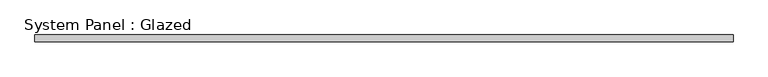
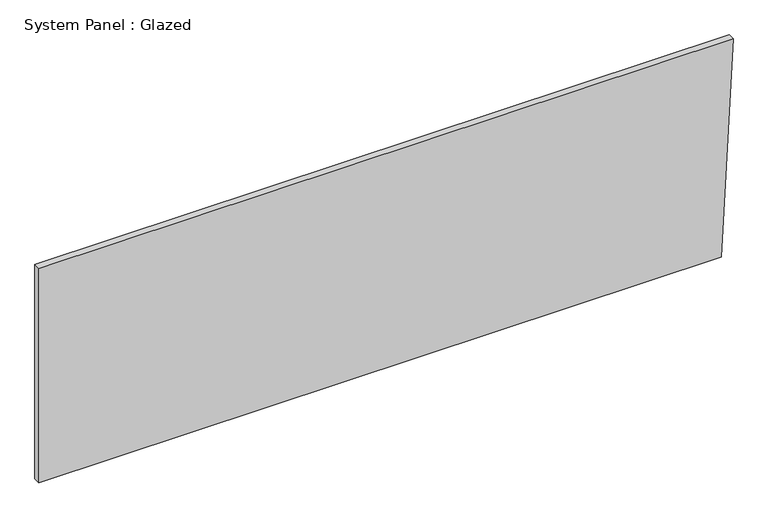
"""IFC4 building model written with IfcOpenShell, lengths in millimetres: plate geometry, System Panel : Glazed."""

import ifcopenshell
import ifcopenshell.guid

model = None  # the IFC model being written
_history = None  # IfcOwnerHistory: only IFC2X3 demands one
_inside = {}  # id of a spatial element -> (the spatial element, [elements in it])
_under = {}  # id of a project, library or spatial element -> (it, [spatial elements below it])
_declared = {}  # id of a project -> (the project, [libraries it declares])
_typed = {}  # id of a type object -> (the type object, [elements of that type])
_made_of = {}  # id of a material, layer set ... -> (it, [elements and type objects made of it])


def new_model(schema):
    """Start an empty IFC model of exactly this schema.

    Asked for "IFC4X3", IfcOpenShell would pick the latest addendum, in which some entities
    have other attributes; the version numbers below select the first issue.
    IFC2X3 requires an IfcOwnerHistory on every rooted entity: one is made here for all.
    """
    global model, _history
    if schema == "IFC4X3":
        model = ifcopenshell.file(schema_version=(4, 3, 0, 0))
    else:
        model = ifcopenshell.file(schema=schema)
    _inside.clear()
    _under.clear()
    _declared.clear()
    _typed.clear()
    _made_of.clear()
    _history = None
    if model.schema == "IFC2X3":
        org = make("IfcOrganization", Name="unknown")
        user = make(
            "IfcPersonAndOrganization",
            ThePerson=make("IfcPerson", FamilyName="unknown"),
            TheOrganization=org,
        )
        app = make(
            "IfcApplication",
            ApplicationDeveloper=org,
            Version="unknown",
            ApplicationFullName="unknown",
            ApplicationIdentifier="unknown",
        )
        _history = make(
            "IfcOwnerHistory",
            OwningUser=user,
            OwningApplication=app,
            ChangeAction="ADDED",
            CreationDate=0,
        )
    return model


def make(cls, **values):
    """One entity of the class cls with the attributes given. An attribute that is None is left unset."""
    return model.create_entity(
        cls, **{name: value for name, value in values.items() if value is not None}
    )


def rooted(cls, **values):
    """An entity with a GlobalId (a new one), such as an element, a storey or a relation."""
    return make(cls, GlobalId=ifcopenshell.guid.new(), OwnerHistory=_history, **values)


def si_unit(unit_type, name, prefix=None):
    """IfcSIUnit, for example si_unit("LENGTHUNIT", "METRE", prefix="MILLI")."""
    return make("IfcSIUnit", UnitType=unit_type, Prefix=prefix, Name=name)


def assignment(units):
    """IfcUnitAssignment: the units of a project."""
    return None if units is None else make("IfcUnitAssignment", Units=units)


def point(xyz):
    """IfcCartesianPoint."""
    return None if xyz is None else make("IfcCartesianPoint", Coordinates=xyz)


def direction(xyz):
    """IfcDirection."""
    return None if xyz is None else make("IfcDirection", DirectionRatios=xyz)


def frame(location, z_axis=None, x_axis=None):
    """IfcAxis2Placement3D, a coordinate frame: its origin and axes. An axis left out is left unset."""
    return make(
        "IfcAxis2Placement3D",
        Location=point(location),
        Axis=direction(z_axis),
        RefDirection=direction(x_axis),
    )


def origin():
    """The frame at (0, 0, 0) with its axes left unset."""
    return frame((0.0, 0.0, 0.0))


def place(relative_to, where):
    """IfcLocalPlacement: puts the frame where relative to a parent placement (None: the world)."""
    return make(
        "IfcLocalPlacement", PlacementRelTo=relative_to, RelativePlacement=where
    )


def context(
    kind, dimensions, precision=None, world=None, true_north=None, identifier=None
):
    """IfcGeometricRepresentationContext, for example the 3D "Model" context."""
    return make(
        "IfcGeometricRepresentationContext",
        ContextIdentifier=identifier,
        ContextType=kind,
        CoordinateSpaceDimension=dimensions,
        Precision=precision,
        WorldCoordinateSystem=world,
        TrueNorth=true_north,
    )


def project(units=None, contexts=None):
    """IfcProject with its units and contexts."""
    return rooted(
        "IfcProject",
        Name="project",
        RepresentationContexts=contexts,
        UnitsInContext=assignment(units),
    )


def spatial(cls, under=None, at=None, **own):
    """A site, building, storey or space (cls), placed at a placement, below another one or the project."""
    s = rooted(cls, ObjectPlacement=at, **own)
    if under is not None:
        _under.setdefault(under.id(), (under, []))[1].append(s)
    return s


def polyline(points):
    """IfcPolyline through the points."""
    return make("IfcPolyline", Points=[point(p) for p in points])


def outline(outer, holes=None, kind="AREA"):
    """IfcArbitraryClosedProfileDef: a profile drawn as a closed curve; with holes, ...WithVoids."""
    if holes is None:
        return make("IfcArbitraryClosedProfileDef", ProfileType=kind, OuterCurve=outer)
    return make(
        "IfcArbitraryProfileDefWithVoids",
        ProfileType=kind,
        OuterCurve=outer,
        InnerCurves=holes,
    )


def extrude(swept, where, along, depth):
    """IfcExtrudedAreaSolid: the profile swept, set in the frame where, extruded along a direction by depth."""
    return make(
        "IfcExtrudedAreaSolid",
        SweptArea=swept,
        Position=where,
        ExtrudedDirection=direction(along),
        Depth=depth,
    )


def shape(context_of_items, identifier, shape_type, items):
    """IfcShapeRepresentation: the items that make up one representation, for example the "Body"."""
    return make(
        "IfcShapeRepresentation",
        ContextOfItems=context_of_items,
        RepresentationIdentifier=identifier,
        RepresentationType=shape_type,
        Items=items,
    )


def source(mapping_origin, context_of_items, identifier, shape_type, items):
    """IfcRepresentationMap: a shape defined once, which mapped items show again and again."""
    return make(
        "IfcRepresentationMap",
        MappingOrigin=mapping_origin,
        MappedRepresentation=shape(context_of_items, identifier, shape_type, items),
    )


def transform(
    local_origin,
    x_axis=None,
    y_axis=None,
    z_axis=None,
    scale=None,
    scale2=None,
    scale3=None,
    uniform=True,
):
    """IfcCartesianTransformationOperator3D, or its non-uniform kind. x_axis, y_axis, z_axis: its Axis1, 2, 3."""
    if uniform:
        return make(
            "IfcCartesianTransformationOperator3D",
            Axis1=direction(x_axis),
            Axis2=direction(y_axis),
            LocalOrigin=point(local_origin),
            Scale=scale,
            Axis3=direction(z_axis),
        )
    return make(
        "IfcCartesianTransformationOperator3DnonUniform",
        Axis1=direction(x_axis),
        Axis2=direction(y_axis),
        LocalOrigin=point(local_origin),
        Scale=scale,
        Axis3=direction(z_axis),
        Scale2=scale2,
        Scale3=scale3,
    )


def mapped(mapping_source, mapping_target):
    """IfcMappedItem: shows the shape of a source again, moved by a transform."""
    return make(
        "IfcMappedItem", MappingSource=mapping_source, MappingTarget=mapping_target
    )


def made_of(thing, what):
    """Note that an element or type object is made of a material, layer set ...; save() writes the relation."""
    if what is not None:
        _made_of.setdefault(what.id(), (what, []))[1].append(thing)
    return thing


def element(
    cls,
    number,
    at=None,
    inside=None,
    cuts=None,
    type_object=None,
    material=None,
    context=None,
    identifier="Body",
    shape_type=None,
    held_by="IfcProductDefinitionShape",
    body=None,
    shapes=None,
    **own,
):
    """One element of the class cls, such as IfcWall. Its Tag is "e" and its number.

    at: its placement. inside: the storey or other place that contains it. cuts: it is an
    opening in that element (IfcRelVoidsElement). A single representation is given by context,
    identifier, shape_type and body (its items); several are given by shapes. held_by: the class
    of the entity that holds the representations. save() writes the other relations.
    """
    e = rooted(cls, Tag="e%d" % number, ObjectPlacement=at, **own)
    if body is not None:
        shapes = [shape(context, identifier, shape_type, body)]
    if shapes is not None:
        e.Representation = make(held_by, Representations=shapes)
    if inside is not None:
        _inside.setdefault(inside.id(), (inside, []))[1].append(e)
    if cuts is not None:
        rooted(
            "IfcRelVoidsElement", RelatingBuildingElement=cuts, RelatedOpeningElement=e
        )
    if type_object is not None:
        _typed.setdefault(type_object.id(), (type_object, []))[1].append(e)
    return made_of(e, material)


def aggregate(whole, parts):
    """IfcRelAggregates: a whole, such as a stair, and the parts it consists of."""
    return rooted("IfcRelAggregates", RelatingObject=whole, RelatedObjects=parts)


def save(model, path):
    """Write the relations noted so far, then the file.

    IfcRelAggregates (storeys below a building ...), IfcRelContainedInSpatialStructure (elements
    in a storey), IfcRelDefinesByType, IfcRelAssociatesMaterial and IfcRelDeclares: one each for
    every whole, place, type object, material and project.
    """
    for whole, parts in _under.values():
        aggregate(whole, parts)
    for where, things in _inside.values():
        rooted(
            "IfcRelContainedInSpatialStructure",
            RelatedElements=things,
            RelatingStructure=where,
        )
    for kind, things in _typed.values():
        rooted("IfcRelDefinesByType", RelatedObjects=things, RelatingType=kind)
    for what, things in _made_of.values():
        rooted("IfcRelAssociatesMaterial", RelatedObjects=things, RelatingMaterial=what)
    for by, libraries in _declared.values():
        rooted("IfcRelDeclares", RelatingContext=by, RelatedDefinitions=libraries)
    model.write(path)


def system_panel_glazed_8e34877b(model_context):
    return source(origin(), model_context, "Body", "SweptSolid", [
        extrude(outline(polyline([(0.0, -1325.8400937), (0.0, 1280.5128872), (866.081558, 1325.8400937), (866.081558, -1325.8400937), (0.0, -1325.8400937)])), frame((0.0, -44.45, 0.0), z_axis=(0.0, 1.0, 0.0), x_axis=(0.0, 0.0, 1.0)), (0.0, 0.0, 1.0), 25.4),
    ])


if __name__ == "__main__":
    model = new_model("IFC4")
    model_context = context("Model", 3, world=origin())
    ifc_project = project(units=[si_unit("LENGTHUNIT", "METRE", prefix="MILLI")], contexts=[model_context])
    site = spatial("IfcSite", under=ifc_project)
    building = spatial("IfcBuilding", under=site)
    placement = place(None, origin())
    system_panel_glazed_shape = system_panel_glazed_8e34877b(model_context)
    element("IfcPlate", 1, ObjectType="System Panel : Glazed", at=placement, inside=building, context=model_context, shape_type="MappedRepresentation", body=[
        mapped(system_panel_glazed_shape, transform((0.0, 0.0, 0.0), x_axis=(1.0, 0.0, 0.0), y_axis=(0.0, 1.0, 0.0), z_axis=(0.0, 0.0, 1.0))),
    ])
    save(model, "model.ifc")

# Revit data of these elements
# Type "System Panel : Glazed"
#   Construction Type Id = "GSP4R"
#   Analytic Construction = "1/8 in Pilkington single glazing"
#   Visual Light Transmittance = 0.9
#   Solar Heat Gain Coefficient = 0.86
#   Heat Transfer Coefficient (U) = 1.18115 BTU/(h·ft²·°F)
#   Define Thermal Properties by = 1
# Element 1 (IfcPlate, "System Panel : Glazed")
#   Materials on its faces: "Glass"
# Materials
#   "Glass": class "Glass", colour RGB 0 128 192, transparency 0.75, Description = "Soda Lime Glass", Cost = 0
